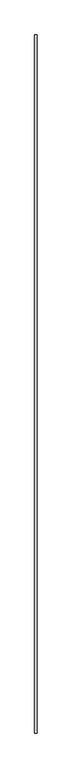
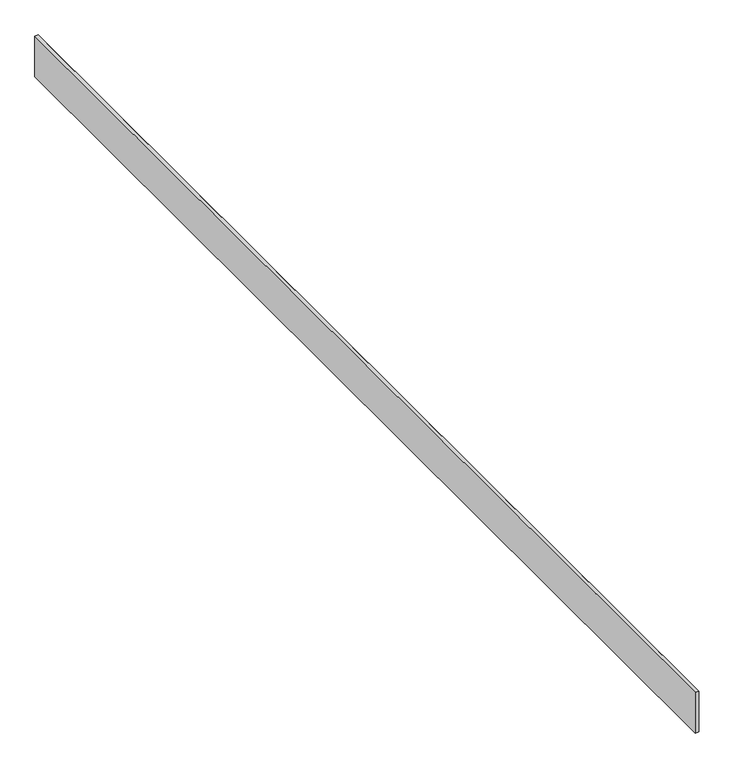
"""IFC4 building model written with IfcOpenShell, lengths in millimetres: proxy geometry, Generic Models 7:Generic Models 1:8:Generic Models 1:8 : Generic Models 7:Generic Models 1:337419:46 : Generic Models 7:Generic Models 1:8:Generic Models 1:8 : Generic Models 7:Generic Models 1:337419:315935."""

from ifc_helpers import new_model, si_unit, frame, origin, place, context, project, spatial, polyline, outline, extrude, source, transform, mapped, element, save


def generic_models_9cf96d4f(model_context):
    return source(origin(), model_context, "Body", "SweptSolid", [
        extrude(outline(polyline([(3903.4402499, 560285.4754749), (3903.4402499, 560270.4117207), (3720.3062499, 560270.4117207), (3720.3062499, 560286.2867207), (3902.6290041, 560286.2867207), (3903.4402499, 560285.4754749)])), frame((0.0, -548060.3163841, 0.0), z_axis=(0.0, 1.0, 0.0), x_axis=(0.0, 0.0, 1.0)), (0.0, 0.0, 1.0), 4876.8),
    ])


if __name__ == "__main__":
    model = new_model("IFC4")
    model_context = context("Model", 3, world=origin())
    ifc_project = project(units=[si_unit("LENGTHUNIT", "METRE", prefix="MILLI")], contexts=[model_context])
    site = spatial("IfcSite", under=ifc_project)
    building = spatial("IfcBuilding", under=site)
    placement = place(None, origin())
    generic_models_shape = generic_models_9cf96d4f(model_context)
    element("IfcBuildingElementProxy", 1, Name="Generic Models 7:Generic Models 1:8:Generic Models 1:8 : Generic Models 7:Generic Models 1:337419:46 : Generic Models 7:Generic Models 1:8:Generic Models 1:8 : Generic Models 7:Generic Models 1:337419:315935", ObjectType="Generic Models 7:Generic Models 1:8:Generic Models 1:8 : Generic Models 7:Generic Models 1:337419:46 : Generic Models 7:Generic Models 1:8:Generic Models 1:8 : Generic Models 7:Generic Models 1:337419:315935", at=placement, inside=building, context=model_context, shape_type="MappedRepresentation", body=[
        mapped(generic_models_shape, transform((0.0, 0.0, 0.0), x_axis=(1.0, 0.0, 0.0), y_axis=(0.0, 1.0, 0.0), z_axis=(0.0, 0.0, 1.0))),
    ])
    save(model, "model.ifc")

# Revit data of these elements
# Type "Generic Models 7:Generic Models 1:8:Generic Models 1:8 : Generic Models 7:Generic Models 1:337419:46 : Generic Models 7:Generic Models 1:8:Generic Models 1:8 : Generic Models 7:Generic Models 1:337419:315935"
#   NameOverride = "Generic Models 7:Generic Models 1:8:Generic Models 1:8 : Generic Models 7:Generic Models 1:337419:315935"
#   ObjectTypeOverride = "Generic Models 1:8 : Generic Models 7:Generic Models 1:337419"
#   Reference = "Generic Models 1"
#   Tag = "315935"
# Element 1 (IfcBuildingElementProxy, "Generic Models 7:Generic Models 1:8:Generic Models 1:8 : Generic Models 7:Generic Models 1:337419:46 : Generic Models 7:Generic Models 1:8:Generic Models 1:8 : Generic Models 7:Generic Models 1:337419:315935")
#   Materials on its faces: "ENGINEERED WOOD TRIM (LP SMARTSIDE)"
# Materials
#   "ENGINEERED WOOD TRIM (LP SMARTSIDE)": class "Wood", colour RGB 108 80 40, transparency 0, Description = "Pinus Echinata", Cost = 0
